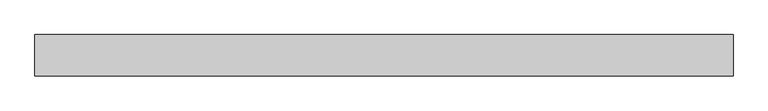
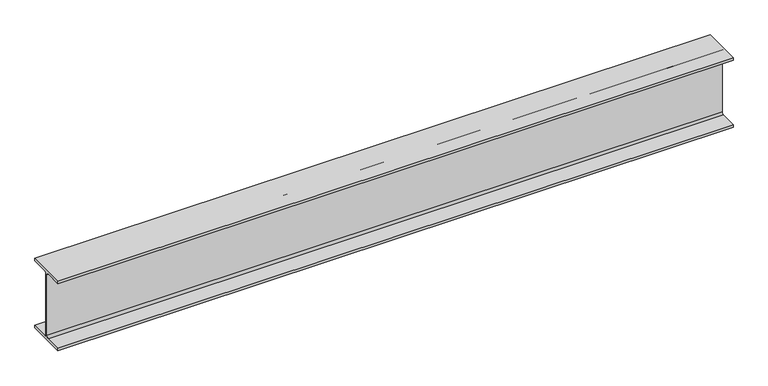
"""IFC4 building model written with IfcOpenShell, lengths in millimetres: beam geometry, Steel Beam_H-KSD3502 : H_SB_ASB_H-250x125x6x9."""

import ifcopenshell
import ifcopenshell.guid

model = None  # the IFC model being written
_history = None  # IfcOwnerHistory: only IFC2X3 demands one
_inside = {}  # id of a spatial element -> (the spatial element, [elements in it])
_under = {}  # id of a project, library or spatial element -> (it, [spatial elements below it])
_declared = {}  # id of a project -> (the project, [libraries it declares])
_typed = {}  # id of a type object -> (the type object, [elements of that type])
_made_of = {}  # id of a material, layer set ... -> (it, [elements and type objects made of it])


def new_model(schema):
    """Start an empty IFC model of exactly this schema.

    Asked for "IFC4X3", IfcOpenShell would pick the latest addendum, in which some entities
    have other attributes; the version numbers below select the first issue.
    IFC2X3 requires an IfcOwnerHistory on every rooted entity: one is made here for all.
    """
    global model, _history
    if schema == "IFC4X3":
        model = ifcopenshell.file(schema_version=(4, 3, 0, 0))
    else:
        model = ifcopenshell.file(schema=schema)
    _inside.clear()
    _under.clear()
    _declared.clear()
    _typed.clear()
    _made_of.clear()
    _history = None
    if model.schema == "IFC2X3":
        org = make("IfcOrganization", Name="unknown")
        user = make(
            "IfcPersonAndOrganization",
            ThePerson=make("IfcPerson", FamilyName="unknown"),
            TheOrganization=org,
        )
        app = make(
            "IfcApplication",
            ApplicationDeveloper=org,
            Version="unknown",
            ApplicationFullName="unknown",
            ApplicationIdentifier="unknown",
        )
        _history = make(
            "IfcOwnerHistory",
            OwningUser=user,
            OwningApplication=app,
            ChangeAction="ADDED",
            CreationDate=0,
        )
    return model


def make(cls, **values):
    """One entity of the class cls with the attributes given. An attribute that is None is left unset."""
    return model.create_entity(
        cls, **{name: value for name, value in values.items() if value is not None}
    )


def rooted(cls, **values):
    """An entity with a GlobalId (a new one), such as an element, a storey or a relation."""
    return make(cls, GlobalId=ifcopenshell.guid.new(), OwnerHistory=_history, **values)


def si_unit(unit_type, name, prefix=None):
    """IfcSIUnit, for example si_unit("LENGTHUNIT", "METRE", prefix="MILLI")."""
    return make("IfcSIUnit", UnitType=unit_type, Prefix=prefix, Name=name)


def assignment(units):
    """IfcUnitAssignment: the units of a project."""
    return None if units is None else make("IfcUnitAssignment", Units=units)


def point(xyz):
    """IfcCartesianPoint."""
    return None if xyz is None else make("IfcCartesianPoint", Coordinates=xyz)


def direction(xyz):
    """IfcDirection."""
    return None if xyz is None else make("IfcDirection", DirectionRatios=xyz)


def frame(location, z_axis=None, x_axis=None):
    """IfcAxis2Placement3D, a coordinate frame: its origin and axes. An axis left out is left unset."""
    return make(
        "IfcAxis2Placement3D",
        Location=point(location),
        Axis=direction(z_axis),
        RefDirection=direction(x_axis),
    )


def frame_2d(location, x_axis=None):
    """IfcAxis2Placement2D, a coordinate frame in the plane: its origin and x axis."""
    return make(
        "IfcAxis2Placement2D", Location=point(location), RefDirection=direction(x_axis)
    )


def origin():
    """The frame at (0, 0, 0) with its axes left unset."""
    return frame((0.0, 0.0, 0.0))


def place(relative_to, where):
    """IfcLocalPlacement: puts the frame where relative to a parent placement (None: the world)."""
    return make(
        "IfcLocalPlacement", PlacementRelTo=relative_to, RelativePlacement=where
    )


def context(
    kind, dimensions, precision=None, world=None, true_north=None, identifier=None
):
    """IfcGeometricRepresentationContext, for example the 3D "Model" context."""
    return make(
        "IfcGeometricRepresentationContext",
        ContextIdentifier=identifier,
        ContextType=kind,
        CoordinateSpaceDimension=dimensions,
        Precision=precision,
        WorldCoordinateSystem=world,
        TrueNorth=true_north,
    )


def project(units=None, contexts=None):
    """IfcProject with its units and contexts."""
    return rooted(
        "IfcProject",
        Name="project",
        RepresentationContexts=contexts,
        UnitsInContext=assignment(units),
    )


def spatial(cls, under=None, at=None, **own):
    """A site, building, storey or space (cls), placed at a placement, below another one or the project."""
    s = rooted(cls, ObjectPlacement=at, **own)
    if under is not None:
        _under.setdefault(under.id(), (under, []))[1].append(s)
    return s


def polyline(points):
    """IfcPolyline through the points."""
    return make("IfcPolyline", Points=[point(p) for p in points])


def circle_curve(where, radius):
    """IfcCircle in the frame where."""
    return make("IfcCircle", Position=where, Radius=radius)


def trimmed(basis, trim1, trim2, sense, master):
    """IfcTrimmedCurve: the piece of a basis curve between two trims."""
    return make(
        "IfcTrimmedCurve",
        BasisCurve=basis,
        Trim1=trim1,
        Trim2=trim2,
        SenseAgreement=sense,
        MasterRepresentation=master,
    )


def segment(curve, same_sense, transition):
    """IfcCompositeCurveSegment."""
    return make(
        "IfcCompositeCurveSegment",
        Transition=transition,
        SameSense=same_sense,
        ParentCurve=curve,
    )


def composite_curve(segments, self_intersect=None):
    """IfcCompositeCurve: segments joined end to end."""
    return make("IfcCompositeCurve", Segments=segments, SelfIntersect=self_intersect)


def outline(outer, holes=None, kind="AREA"):
    """IfcArbitraryClosedProfileDef: a profile drawn as a closed curve; with holes, ...WithVoids."""
    if holes is None:
        return make("IfcArbitraryClosedProfileDef", ProfileType=kind, OuterCurve=outer)
    return make(
        "IfcArbitraryProfileDefWithVoids",
        ProfileType=kind,
        OuterCurve=outer,
        InnerCurves=holes,
    )


def extrude(swept, where, along, depth):
    """IfcExtrudedAreaSolid: the profile swept, set in the frame where, extruded along a direction by depth."""
    return make(
        "IfcExtrudedAreaSolid",
        SweptArea=swept,
        Position=where,
        ExtrudedDirection=direction(along),
        Depth=depth,
    )


def shape(context_of_items, identifier, shape_type, items):
    """IfcShapeRepresentation: the items that make up one representation, for example the "Body"."""
    return make(
        "IfcShapeRepresentation",
        ContextOfItems=context_of_items,
        RepresentationIdentifier=identifier,
        RepresentationType=shape_type,
        Items=items,
    )


def source(mapping_origin, context_of_items, identifier, shape_type, items):
    """IfcRepresentationMap: a shape defined once, which mapped items show again and again."""
    return make(
        "IfcRepresentationMap",
        MappingOrigin=mapping_origin,
        MappedRepresentation=shape(context_of_items, identifier, shape_type, items),
    )


def transform(
    local_origin,
    x_axis=None,
    y_axis=None,
    z_axis=None,
    scale=None,
    scale2=None,
    scale3=None,
    uniform=True,
):
    """IfcCartesianTransformationOperator3D, or its non-uniform kind. x_axis, y_axis, z_axis: its Axis1, 2, 3."""
    if uniform:
        return make(
            "IfcCartesianTransformationOperator3D",
            Axis1=direction(x_axis),
            Axis2=direction(y_axis),
            LocalOrigin=point(local_origin),
            Scale=scale,
            Axis3=direction(z_axis),
        )
    return make(
        "IfcCartesianTransformationOperator3DnonUniform",
        Axis1=direction(x_axis),
        Axis2=direction(y_axis),
        LocalOrigin=point(local_origin),
        Scale=scale,
        Axis3=direction(z_axis),
        Scale2=scale2,
        Scale3=scale3,
    )


def mapped(mapping_source, mapping_target):
    """IfcMappedItem: shows the shape of a source again, moved by a transform."""
    return make(
        "IfcMappedItem", MappingSource=mapping_source, MappingTarget=mapping_target
    )


def made_of(thing, what):
    """Note that an element or type object is made of a material, layer set ...; save() writes the relation."""
    if what is not None:
        _made_of.setdefault(what.id(), (what, []))[1].append(thing)
    return thing


def element(
    cls,
    number,
    at=None,
    inside=None,
    cuts=None,
    type_object=None,
    material=None,
    context=None,
    identifier="Body",
    shape_type=None,
    held_by="IfcProductDefinitionShape",
    body=None,
    shapes=None,
    **own,
):
    """One element of the class cls, such as IfcWall. Its Tag is "e" and its number.

    at: its placement. inside: the storey or other place that contains it. cuts: it is an
    opening in that element (IfcRelVoidsElement). A single representation is given by context,
    identifier, shape_type and body (its items); several are given by shapes. held_by: the class
    of the entity that holds the representations. save() writes the other relations.
    """
    e = rooted(cls, Tag="e%d" % number, ObjectPlacement=at, **own)
    if body is not None:
        shapes = [shape(context, identifier, shape_type, body)]
    if shapes is not None:
        e.Representation = make(held_by, Representations=shapes)
    if inside is not None:
        _inside.setdefault(inside.id(), (inside, []))[1].append(e)
    if cuts is not None:
        rooted(
            "IfcRelVoidsElement", RelatingBuildingElement=cuts, RelatedOpeningElement=e
        )
    if type_object is not None:
        _typed.setdefault(type_object.id(), (type_object, []))[1].append(e)
    return made_of(e, material)


def aggregate(whole, parts):
    """IfcRelAggregates: a whole, such as a stair, and the parts it consists of."""
    return rooted("IfcRelAggregates", RelatingObject=whole, RelatedObjects=parts)


def save(model, path):
    """Write the relations noted so far, then the file.

    IfcRelAggregates (storeys below a building ...), IfcRelContainedInSpatialStructure (elements
    in a storey), IfcRelDefinesByType, IfcRelAssociatesMaterial and IfcRelDeclares: one each for
    every whole, place, type object, material and project.
    """
    for whole, parts in _under.values():
        aggregate(whole, parts)
    for where, things in _inside.values():
        rooted(
            "IfcRelContainedInSpatialStructure",
            RelatedElements=things,
            RelatingStructure=where,
        )
    for kind, things in _typed.values():
        rooted("IfcRelDefinesByType", RelatedObjects=things, RelatingType=kind)
    for what, things in _made_of.values():
        rooted("IfcRelAssociatesMaterial", RelatedObjects=things, RelatingMaterial=what)
    for by, libraries in _declared.values():
        rooted("IfcRelDeclares", RelatingContext=by, RelatedDefinitions=libraries)
    model.write(path)


def beam_b704906e(model_context):
    return source(origin(), model_context, "Body", "SweptSolid", [
        extrude(outline(composite_curve([segment(polyline([(82.5, -141.5), (82.5, -151.7), (-82.5, -151.7), (-82.5, -141.5), (-11.9, -141.5)]), True, "CONTINUOUS"), segment(trimmed(circle_curve(frame_2d((-11.9, -132.6)), 8.9), [point((-11.9, -141.5))], [point((-3.0, -132.6))], True, "CARTESIAN"), True, "CONTINUOUS"), segment(polyline([(-3.0, -132.6), (-3.0, 132.6)]), True, "CONTINUOUS"), segment(trimmed(circle_curve(frame_2d((-11.9, 132.6)), 8.9), [point((-3.0, 132.6))], [point((-11.9, 141.5))], True, "CARTESIAN"), True, "CONTINUOUS"), segment(polyline([(-11.9, 141.5), (-82.5, 141.5), (-82.5, 151.7), (82.5, 151.7), (82.5, 141.5), (11.9, 141.5)]), True, "CONTINUOUS"), segment(trimmed(circle_curve(frame_2d((11.9, 132.6)), 8.9), [point((11.9, 141.5))], [point((3.0, 132.6))], True, "CARTESIAN"), True, "CONTINUOUS"), segment(polyline([(3.0, 132.6), (3.0, -132.6)]), True, "CONTINUOUS"), segment(trimmed(circle_curve(frame_2d((11.9, -132.6)), 8.9), [point((3.0, -132.6))], [point((11.9, -141.5))], True, "CARTESIAN"), True, "CONTINUOUS"), segment(polyline([(11.9, -141.5), (82.5, -141.5)]), True, "CONTINUOUS")], self_intersect=False)), frame((-1382.298157, 0.0, 0.0), z_axis=(1.0, 0.0, 0.0), x_axis=(0.0, 1.0, 0.0)), (0.0, 0.0, 1.0), 2794.5982),
    ])


if __name__ == "__main__":
    model = new_model("IFC4")
    model_context = context("Model", 3, world=origin())
    ifc_project = project(units=[si_unit("LENGTHUNIT", "METRE", prefix="MILLI")], contexts=[model_context])
    site = spatial("IfcSite", under=ifc_project)
    building = spatial("IfcBuilding", under=site)
    placement = place(None, origin())
    beam_shape = beam_b704906e(model_context)
    element("IfcBeam", 1, ObjectType="Steel Beam_H-KSD3502 : H_SB_ASB_H-250x125x6x9", at=placement, inside=building, context=model_context, shape_type="MappedRepresentation", body=[
        mapped(beam_shape, transform((0.0, 0.0, 0.0), x_axis=(1.0, 0.0, 0.0), y_axis=(0.0, 1.0, 0.0), z_axis=(0.0, 0.0, 1.0))),
    ])
    save(model, "model.ifc")

# Revit data of these elements
# Type "Steel Beam_H-KSD3502 : H_SB_ASB_H-250x125x6x9"
#   Width = 12.5 cm
#   Web Thickness = 0.6 cm
#   Web Fillet = 1.2 cm
#   Warping Constant = 42539.8 cm⁶
#   Torsional Moment of Inertia = 7.8102 cm⁴
#   Torsional Modulus = 1.0 cm³
#   Section Area = 37.66 cm²
#   Plastic Modulus weak axis = 73.1 cm³
#   Plastic Modulus strong axis = 366.0 cm³
#   Perimeter = 0.97 m²/m
#   Nominal Weight = 29.60 kgf/m
#   Moment of Inertia weak axis = 294.00 cm⁴
#   Moment of Inertia strong axis = 4050.00 cm⁴
#   Height = 25.0 cm
#   Flange Thickness = 0.9 cm
#   Elastic Modulus weak axis = 47.0 cm³
#   Elastic Modulus strong axis = 324.0 cm³
#   Centroid Vertical = 12.5 cm
#   Centroid Horizontal = 6.25 cm
#   Length [instance default] = 1.5240 m
#   Structural Material [instance default] = Steel, 45-345
#   Assembly Code = ""
# Element 1 (IfcBeam, "Steel Beam_H-KSD3502 : H_SB_ASB_H-250x125x6x9")
#   Structural Material = none
# Materials
#   "Steel, 45-345": class "Metal", colour RGB 189 187 185, transparency 0, Description = "Steel 345 MPa", Cost = 0
